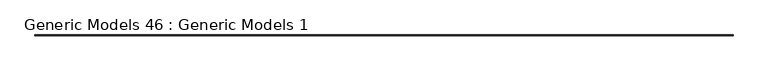
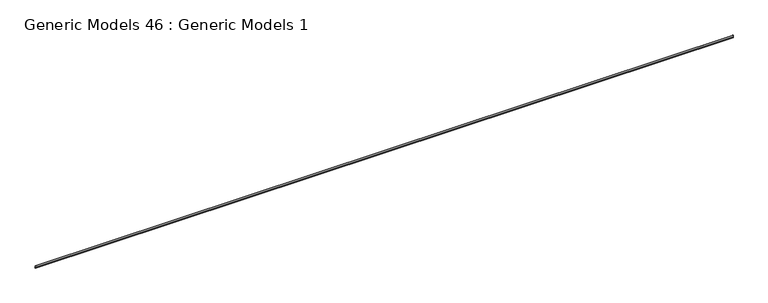
"""IFC4 building model written with IfcOpenShell, lengths in millimetres: proxy geometry, Generic Models 46 : Generic Models 1."""

from ifc_helpers import new_model, si_unit, frame, origin, place, context, project, spatial, polyline, outline, extrude, source, transform, mapped, element, save


def generic_models_46_generic_models_1_6bd6e951(model_context):
    return source(origin(), model_context, "Body", "SweptSolid", [
        extrude(outline(polyline([(14304.5225836, 126996.7728942), (14284.368967, 126990.2949461), (14283.5456461, 126985.9229543), (14282.2975836, 126986.1579859), (14283.2607787, 126991.2727363), (14300.3723813, 126996.7728942), (14282.2975836, 127002.5826506), (14282.2975836, 127047.5728942), (14283.5675836, 127047.5728942), (14283.5675836, 127003.50843), (14304.5225836, 126996.7728942)])), frame((-20998.9733045, 0.0, 0.0), z_axis=(1.0, 0.0, 0.0), x_axis=(0.0, 1.0, 0.0)), (0.0, 0.0, 1.0), 19050.0),
    ])


if __name__ == "__main__":
    model = new_model("IFC4")
    model_context = context("Model", 3, world=origin())
    ifc_project = project(units=[si_unit("LENGTHUNIT", "METRE", prefix="MILLI")], contexts=[model_context])
    site = spatial("IfcSite", under=ifc_project)
    building = spatial("IfcBuilding", under=site)
    placement = place(None, origin())
    generic_models_46_generic_models_1_shape = generic_models_46_generic_models_1_6bd6e951(model_context)
    element("IfcBuildingElementProxy", 1, Name="Generic Models 46 : Generic Models 1", ObjectType="Generic Models 46 : Generic Models 1", at=placement, inside=building, context=model_context, shape_type="MappedRepresentation", body=[
        mapped(generic_models_46_generic_models_1_shape, transform((0.0, 0.0, 0.0), x_axis=(1.0, 0.0, 0.0), y_axis=(0.0, 1.0, 0.0), z_axis=(0.0, 0.0, 1.0))),
    ])
    save(model, "model.ifc")

# Revit data of these elements
# Element 1 (IfcBuildingElementProxy, "Generic Models 46 : Generic Models 1")
#   Materials on its faces: "_16 GA. COPPER WEEP SCREED W/ MIN. 3 1/2\" ATTACHEMENT FLANGE - LAP UNDERLAYMENT OVER WEED SCREED"
# Materials
#   "_16 GA. COPPER WEEP SCREED W/ MIN. 3 1/2\" ATTACHEMENT FLANGE - LAP UNDERLAYMENT OVER WEED SCREED": class "Generic", colour RGB 253 192 103, transparency 0, Cost = 0
